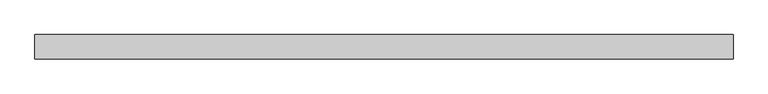
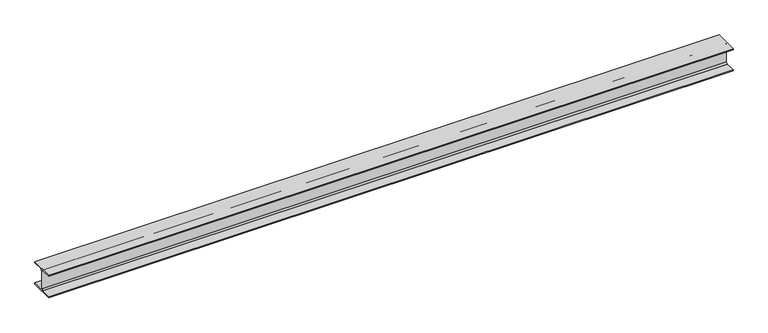
"""IFC4 building model written with IfcOpenShell, lengths in millimetres: beam geometry, 0912_Steel Framing_H-KSD3502 : H_SB_ASB_H-300x300x10x15."""

from ifc_helpers import new_model, si_unit, point, frame, frame_2d, origin, place, context, project, spatial, polyline, circle_curve, trimmed, segment, composite_curve, outline, extrude, source, transform, mapped, element, save


def beam_0b62dadb(model_context):
    return source(origin(), model_context, "Body", "SweptSolid", [
        extrude(outline(composite_curve([segment(polyline([(150.0, -135.0), (150.0, -150.0), (-150.0, -150.0), (-150.0, -135.0), (-23.0, -135.0)]), True, "CONTINUOUS"), segment(trimmed(circle_curve(frame_2d((-23.0, -117.0)), 18.0), [point((-23.0, -135.0))], [point((-5.0, -117.0))], True, "CARTESIAN"), True, "CONTINUOUS"), segment(polyline([(-5.0, -117.0), (-5.0, 117.0)]), True, "CONTINUOUS"), segment(trimmed(circle_curve(frame_2d((-23.0, 117.0)), 18.0), [point((-5.0, 117.0))], [point((-23.0, 135.0))], True, "CARTESIAN"), True, "CONTINUOUS"), segment(polyline([(-23.0, 135.0), (-150.0, 135.0), (-150.0, 150.0), (150.0, 150.0), (150.0, 135.0), (23.0, 135.0)]), True, "CONTINUOUS"), segment(trimmed(circle_curve(frame_2d((23.0, 117.0)), 18.0), [point((23.0, 135.0))], [point((5.0, 117.0))], True, "CARTESIAN"), True, "CONTINUOUS"), segment(polyline([(5.0, 117.0), (5.0, -117.0)]), True, "CONTINUOUS"), segment(trimmed(circle_curve(frame_2d((23.0, -117.0)), 18.0), [point((5.0, -117.0))], [point((23.0, -135.0))], True, "CARTESIAN"), True, "CONTINUOUS"), segment(polyline([(23.0, -135.0), (150.0, -135.0)]), True, "CONTINUOUS")], self_intersect=False)), frame((-4374.2452733, 0.0, 0.0), z_axis=(1.0, 0.0, 0.0), x_axis=(0.0, 1.0, 0.0)), (0.0, 0.0, 1.0), 8647.1704515),
    ])


if __name__ == "__main__":
    model = new_model("IFC4")
    model_context = context("Model", 3, world=origin())
    ifc_project = project(units=[si_unit("LENGTHUNIT", "METRE", prefix="MILLI")], contexts=[model_context])
    site = spatial("IfcSite", under=ifc_project)
    building = spatial("IfcBuilding", under=site)
    placement = place(None, origin())
    beam_shape = beam_0b62dadb(model_context)
    element("IfcBeam", 1, ObjectType="0912_Steel Framing_H-KSD3502 : H_SB_ASB_H-300x300x10x15", at=placement, inside=building, context=model_context, shape_type="MappedRepresentation", body=[
        mapped(beam_shape, transform((0.0, 0.0, 0.0), x_axis=(1.0, 0.0, 0.0), y_axis=(0.0, 1.0, 0.0), z_axis=(0.0, 0.0, 1.0))),
    ])
    save(model, "model.ifc")

# Revit data of these elements
# Type "0912_Steel Framing_H-KSD3502 : H_SB_ASB_H-300x300x10x15"
#   H_WM Code_1 = "S01AA001-00001 | Main Steel Structure Fabrication Work | Shelter/Building | Heavy Steel - Standard (Weight≥90KG/M) | Material: (   )"
#   H_WM Code_2 = "S03AA027-00001 | Main Steel Structure Erection Work | Shelter/Building | Heavy Steel (Weight≥90KG/M) | Material: (   )"
#   H_WM Code_3 = "S01AA010-00001 | Main Steel Structure Fabrication Work | Shelter/Building | Steel Painting/Coating | for Non-Fireproofed Steel Surface, Surface Preparation, Primer, Second & Final Coat | Material: (   )"
#   H_Q'ty Cal Type Tag = "SB-Q2"
#   Width = 30.0 cm
#   Web Thickness = 1.0 cm
#   Web Fillet = 1.8 cm
#   Warping Constant = 1370000.0 cm⁶
#   W = 0
#   Torsional Moment of Inertia = 77.00 cm⁴
#   Section Area = 119.8 cm²
#   Plastic Modulus weak axis = 684.0 cm³
#   Plastic Modulus strong axis = 1500.0 cm³
#   Perimeter = 1.75 m²/m
#   Nominal Weight = 94.00 kgf/m
#   Moment of Inertia weak axis = 6750.00 cm⁴
#   Moment of Inertia strong axis = 20400.00 cm⁴
#   Height = 30.0 cm
#   Flange Thickness = 1.5 cm
#   Elastic Modulus weak axis = 450.0 cm³
#   Elastic Modulus strong axis = 1360.0 cm³
#   Centroid Vertical = 15.0 cm
#   Centroid Horizontal = 15.0 cm
#   Ix = 204000000
#   Length [instance default] = 1.5240 m
#   Zx = 1500000
#   b = 0.3000 m
#   h = 0.3000 m
#   r = 0.0180 m
#   s = 0.0100 m
#   t = 0.0150 m
#   A = 0.01198 m²
#   Structural Material [instance default] = Steel, 45-345
#   Assembly Code = ""
# Element 1 (IfcBeam, "0912_Steel Framing_H-KSD3502 : H_SB_ASB_H-300x300x10x15")
#   Structural Material = none
# Materials
#   "Steel, 45-345": class "Metal", colour RGB 189 187 185, transparency 0, Description = "Steel 345 MPa", Cost = 0
